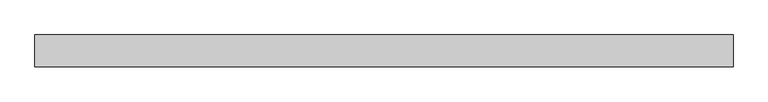
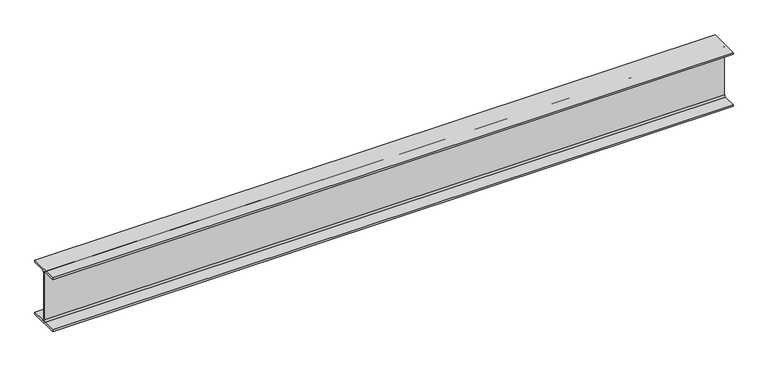
"""IFC4 building model written with IfcOpenShell, lengths in millimetres: beam geometry, Steel Beam_H-KSD3502 : H_SB_ASB_H-200x200x8x12."""

from ifc_helpers import new_model, si_unit, point, frame, frame_2d, origin, place, context, project, spatial, polyline, circle_curve, trimmed, segment, composite_curve, outline, extrude, source, transform, mapped, element, save


def beam_a769b179(model_context):
    return source(origin(), model_context, "Body", "SweptSolid", [
        extrude(outline(composite_curve([segment(polyline([(82.5, -141.5), (82.5, -151.7), (-82.5, -151.7), (-82.5, -141.5), (-11.9, -141.5)]), True, "CONTINUOUS"), segment(trimmed(circle_curve(frame_2d((-11.9, -132.6)), 8.9), [point((-11.9, -141.5))], [point((-3.0, -132.6))], True, "CARTESIAN"), True, "CONTINUOUS"), segment(polyline([(-3.0, -132.6), (-3.0, 132.6)]), True, "CONTINUOUS"), segment(trimmed(circle_curve(frame_2d((-11.9, 132.6)), 8.9), [point((-3.0, 132.6))], [point((-11.9, 141.5))], True, "CARTESIAN"), True, "CONTINUOUS"), segment(polyline([(-11.9, 141.5), (-82.5, 141.5), (-82.5, 151.7), (82.5, 151.7), (82.5, 141.5), (11.9, 141.5)]), True, "CONTINUOUS"), segment(trimmed(circle_curve(frame_2d((11.9, 132.6)), 8.9), [point((11.9, 141.5))], [point((3.0, 132.6))], True, "CARTESIAN"), True, "CONTINUOUS"), segment(polyline([(3.0, 132.6), (3.0, -132.6)]), True, "CONTINUOUS"), segment(trimmed(circle_curve(frame_2d((11.9, -132.6)), 8.9), [point((3.0, -132.6))], [point((11.9, -141.5))], True, "CARTESIAN"), True, "CONTINUOUS"), segment(polyline([(11.9, -141.5), (82.5, -141.5)]), True, "CONTINUOUS")], self_intersect=False)), frame((-1907.7947202, 0.0, 0.0), z_axis=(1.0, 0.0, 0.0), x_axis=(0.0, 1.0, 0.0)), (0.0, 0.0, 1.0), 3628.373533),
    ])


if __name__ == "__main__":
    model = new_model("IFC4")
    model_context = context("Model", 3, world=origin())
    ifc_project = project(units=[si_unit("LENGTHUNIT", "METRE", prefix="MILLI")], contexts=[model_context])
    site = spatial("IfcSite", under=ifc_project)
    building = spatial("IfcBuilding", under=site)
    placement = place(None, origin())
    beam_shape = beam_a769b179(model_context)
    element("IfcBeam", 1, ObjectType="Steel Beam_H-KSD3502 : H_SB_ASB_H-200x200x8x12", at=placement, inside=building, context=model_context, shape_type="MappedRepresentation", body=[
        mapped(beam_shape, transform((0.0, 0.0, 0.0), x_axis=(1.0, 0.0, 0.0), y_axis=(0.0, 1.0, 0.0), z_axis=(0.0, 0.0, 1.0))),
    ])
    save(model, "model.ifc")

# Revit data of these elements
# Type "Steel Beam_H-KSD3502 : H_SB_ASB_H-200x200x8x12"
#   Width = 20.0 cm
#   Web Thickness = 0.8 cm
#   Web Fillet = 1.3 cm
#   Warping Constant = 141376.0 cm⁶
#   Torsional Moment of Inertia = 26.2485 cm⁴
#   Torsional Modulus = 1.0 cm³
#   Section Area = 63.53 cm²
#   Plastic Modulus weak axis = 244.0 cm³
#   Plastic Modulus strong axis = 525.0 cm³
#   Perimeter = 1.16 m²/m
#   Nominal Weight = 49.90 kgf/m
#   Moment of Inertia weak axis = 1600.00 cm⁴
#   Moment of Inertia strong axis = 4720.00 cm⁴
#   Height = 20.0 cm
#   Flange Thickness = 1.2 cm
#   Elastic Modulus weak axis = 160.0 cm³
#   Elastic Modulus strong axis = 472.0 cm³
#   Centroid Vertical = 10.0 cm
#   Centroid Horizontal = 10.0 cm
#   Length [instance default] = 1.5240 m
#   Structural Material [instance default] = Steel, 45-345
#   Assembly Code = ""
# Element 1 (IfcBeam, "Steel Beam_H-KSD3502 : H_SB_ASB_H-200x200x8x12")
#   Structural Material = none
# Materials
#   "Steel, 45-345": class "Metal", colour RGB 189 187 185, transparency 0, Description = "Steel 345 MPa", Cost = 0
